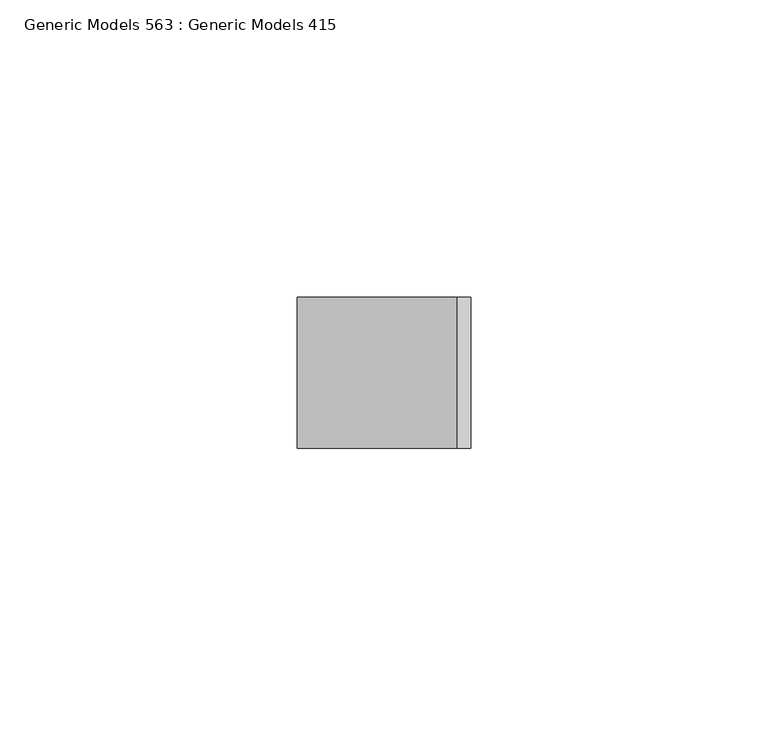
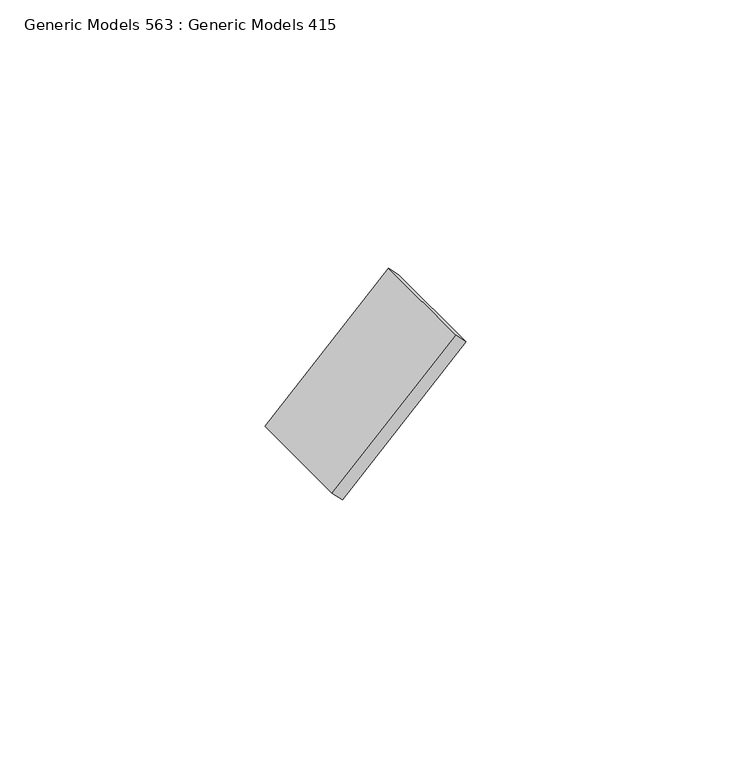
"""IFC4 building model written with IfcOpenShell, lengths in millimetres: proxy geometry, Generic Models 563 : Generic Models 415."""

from ifc_helpers import new_model, si_unit, frame, origin, place, context, project, spatial, polyline, outline, extrude, source, transform, mapped, element, save


def generic_models_563_generic_models_415_49dee8cf(model_context):
    return source(origin(), model_context, "Body", "SweptSolid", [
        extrude(outline(polyline([(0.0, -3.175), (0.0, 0.0), (25.4, 0.0), (25.4, -3.175), (0.0, -3.175)])), frame((7848.0411784, 4501.3863946, 124305.3849742), z_axis=(0.7071067811867181, 0.0, 0.707106781186377), x_axis=(0.0, -1.0, 0.0)), (0.0, 0.0, 1.0), 38.1),
    ])


if __name__ == "__main__":
    model = new_model("IFC4")
    model_context = context("Model", 3, world=origin())
    ifc_project = project(units=[si_unit("LENGTHUNIT", "METRE", prefix="MILLI")], contexts=[model_context])
    site = spatial("IfcSite", under=ifc_project)
    building = spatial("IfcBuilding", under=site)
    placement = place(None, origin())
    generic_models_563_generic_models_415_shape = generic_models_563_generic_models_415_49dee8cf(model_context)
    element("IfcBuildingElementProxy", 1, Name="Generic Models 563 : Generic Models 415", ObjectType="Generic Models 563 : Generic Models 415", at=placement, inside=building, context=model_context, shape_type="MappedRepresentation", body=[
        mapped(generic_models_563_generic_models_415_shape, transform((0.0, 0.0, 0.0), x_axis=(1.0, 0.0, 0.0), y_axis=(0.0, 1.0, 0.0), z_axis=(0.0, 0.0, 1.0))),
    ])
    save(model, "model.ifc")

# Revit data of these elements
# Element 1 (IfcBuildingElementProxy, "Generic Models 563 : Generic Models 415")
#   Materials on its faces: "_WELDED STEEL TABS FOR LOUVER ATTACHMENT"
# Materials
#   "_WELDED STEEL TABS FOR LOUVER ATTACHMENT": class "Metal", colour RGB 199 199 199, transparency 0, Description = "Structural steel 50ksi", Cost = 0
